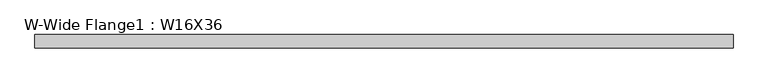
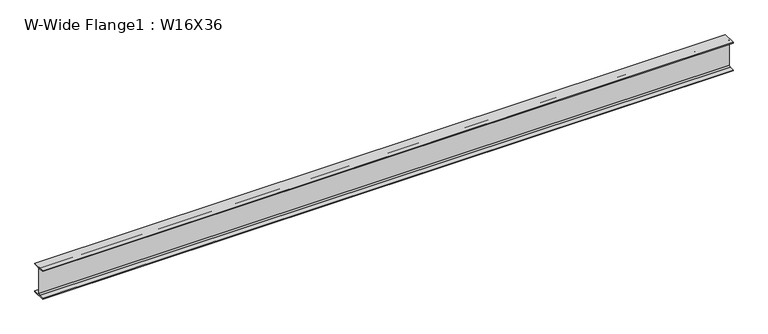
"""IFC4 building model written with IfcOpenShell, lengths in millimetres: beam geometry, W-Wide Flange1 : W16X36."""

from ifc_helpers import new_model, si_unit, point, frame, frame_2d, origin, place, context, project, spatial, polyline, circle_curve, trimmed, segment, composite_curve, outline, extrude, source, transform, mapped, element, save


def w_wide_flange1_w16x36_6552f6d8(model_context):
    return source(origin(), model_context, "Body", "SweptSolid", [
        extrude(outline(composite_curve([segment(polyline([(88.773, -191.008), (88.773, -201.93), (-88.773, -201.93), (-88.773, -191.008), (-21.3995, -191.008)]), True, "CONTINUOUS"), segment(trimmed(circle_curve(frame_2d((-21.3995, -173.355)), 17.653), [point((-21.3995, -191.008))], [point((-3.7465, -173.355))], True, "CARTESIAN"), True, "CONTINUOUS"), segment(polyline([(-3.7465, -173.355), (-3.7465, 173.355)]), True, "CONTINUOUS"), segment(trimmed(circle_curve(frame_2d((-21.3995, 173.355)), 17.653), [point((-3.7465, 173.355))], [point((-21.3995, 191.008))], True, "CARTESIAN"), True, "CONTINUOUS"), segment(polyline([(-21.3995, 191.008), (-88.773, 191.008), (-88.773, 201.93), (88.773, 201.93), (88.773, 191.008), (21.3995, 191.008)]), True, "CONTINUOUS"), segment(trimmed(circle_curve(frame_2d((21.3995, 173.355)), 17.653), [point((21.3995, 191.008))], [point((3.7465, 173.355))], True, "CARTESIAN"), True, "CONTINUOUS"), segment(polyline([(3.7465, 173.355), (3.7465, -173.355)]), True, "CONTINUOUS"), segment(trimmed(circle_curve(frame_2d((21.3995, -173.355)), 17.653), [point((3.7465, -173.355))], [point((21.3995, -191.008))], True, "CARTESIAN"), True, "CONTINUOUS"), segment(polyline([(21.3995, -191.008), (88.773, -191.008)]), True, "CONTINUOUS")], self_intersect=False)), frame((-4649.5235692, 0.0, 0.0), z_axis=(1.0, 0.0, 0.0), x_axis=(0.0, 1.0, 0.0)), (0.0, 0.0, 1.0), 9285.2688734),
    ])


if __name__ == "__main__":
    model = new_model("IFC4")
    model_context = context("Model", 3, world=origin())
    ifc_project = project(units=[si_unit("LENGTHUNIT", "METRE", prefix="MILLI")], contexts=[model_context])
    site = spatial("IfcSite", under=ifc_project)
    building = spatial("IfcBuilding", under=site)
    placement = place(None, origin())
    w_wide_flange1_w16x36_shape = w_wide_flange1_w16x36_6552f6d8(model_context)
    element("IfcBeam", 1, ObjectType="W-Wide Flange1 : W16X36", at=placement, inside=building, context=model_context, shape_type="MappedRepresentation", body=[
        mapped(w_wide_flange1_w16x36_shape, transform((0.0, 0.0, 0.0), x_axis=(1.0, 0.0, 0.0), y_axis=(0.0, 1.0, 0.0), z_axis=(0.0, 0.0, 1.0))),
    ])
    save(model, "model.ifc")

# Revit data of these elements
# Type "W-Wide Flange1 : W16X36"
#   Assembly Code = "B10"
#   W = 36
#   Start Extension Calculation [instance default] = 10' - 0"
#   Start Extension [instance default] = -0' - 0 1/2"
#   End Extension Calculation [instance default] = 10' - 0"
#   End Extension [instance default] = -0' - 0 1/2"
#   Length [instance default] = 5' - 0"
#   bf = 0' - 6.99"
#   d = 1' - 3.9"
#   k = 0' - 1 1/8"
#   k2 = 0' - 0.695"
#   tf = 0' - 0.43"
#   tw = 0' - 0.295"
#   A = 0.0736111 SF
#   Structural Material [instance default] = Metal - Steel - ASTM A992
# Element 1 (IfcBeam, "W-Wide Flange1 : W16X36")
#   Materials on its faces: "Metal - Steel - ASTM A992"
# Materials
#   "Metal - Steel - ASTM A992": class "Metal", colour RGB 199 199 199, transparency 0
